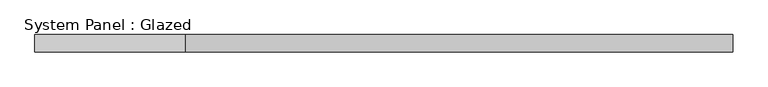
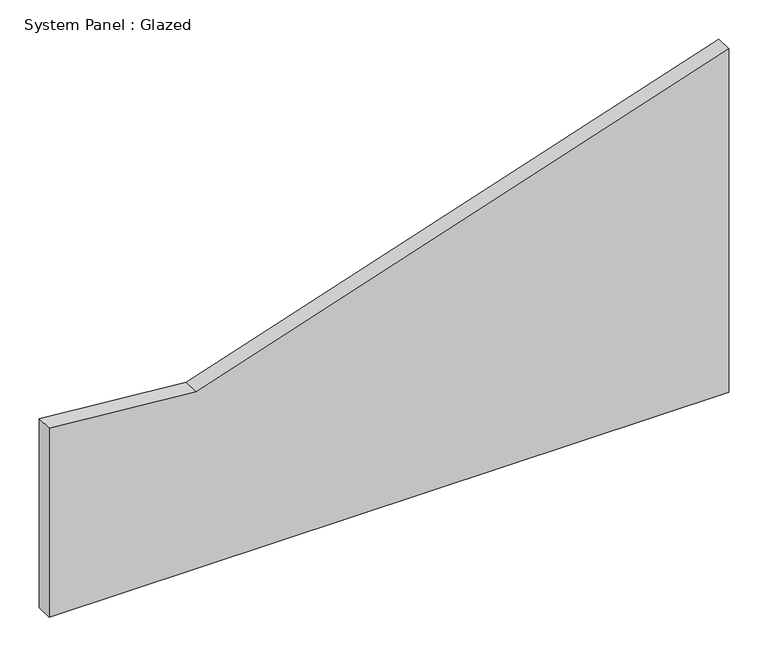
"""IFC4 building model written with IfcOpenShell, lengths in millimetres: plate geometry, System Panel : Glazed."""

from ifc_helpers import new_model, si_unit, frame, origin, place, context, project, spatial, polyline, outline, extrude, source, transform, mapped, element, save


def system_panel_glazed_fbbcfb18(model_context):
    return source(origin(), model_context, "Body", "SweptSolid", [
        extrude(outline(polyline([(0.0, -500.0), (0.0, 500.0), (534.1300252, 500.0), (275.0273689, -283.6395573), (294.0824743, -500.0), (0.0, -500.0)])), frame((0.0, 24.5, 0.0), z_axis=(0.0, 1.0, 0.0), x_axis=(0.0, 0.0, 1.0)), (0.0, 0.0, 1.0), 25.0),
    ])


if __name__ == "__main__":
    model = new_model("IFC4")
    model_context = context("Model", 3, world=origin())
    ifc_project = project(units=[si_unit("LENGTHUNIT", "METRE", prefix="MILLI")], contexts=[model_context])
    site = spatial("IfcSite", under=ifc_project)
    building = spatial("IfcBuilding", under=site)
    placement = place(None, origin())
    system_panel_glazed_shape = system_panel_glazed_fbbcfb18(model_context)
    element("IfcPlate", 1, ObjectType="System Panel : Glazed", at=placement, inside=building, context=model_context, shape_type="MappedRepresentation", body=[
        mapped(system_panel_glazed_shape, transform((0.0, 0.0, 0.0), x_axis=(1.0, 0.0, 0.0), y_axis=(0.0, 1.0, 0.0), z_axis=(0.0, 0.0, 1.0))),
    ])
    save(model, "model.ifc")

# Revit data of these elements
# Element 1 (IfcPlate, "System Panel : Glazed")
#   Materials on its faces: "Glass"
# Materials
#   "Glass": class "Glass", colour RGB 218 227 224, transparency 0.85, Description = "Soda Lime Glass", Cost = 0
